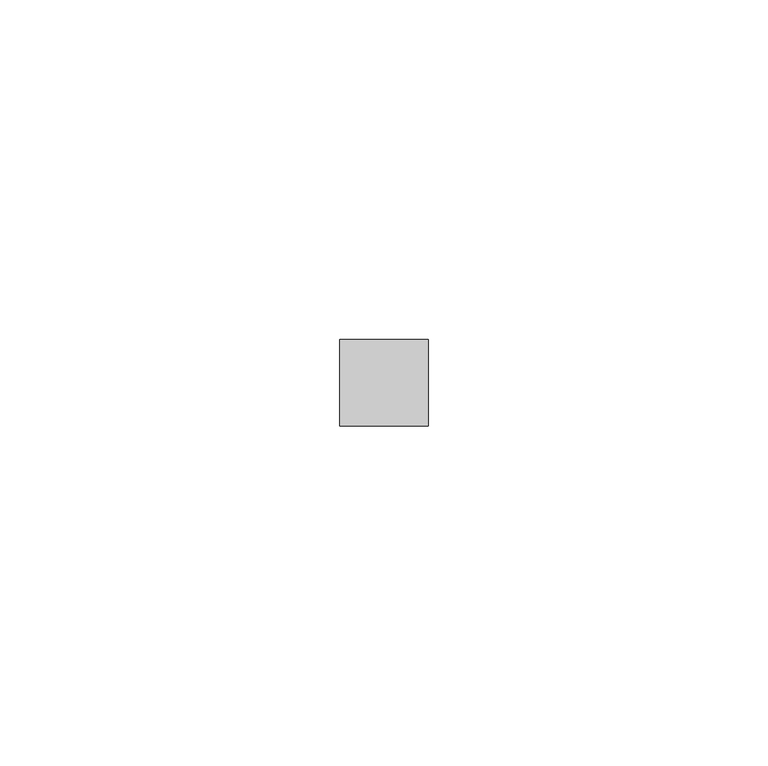
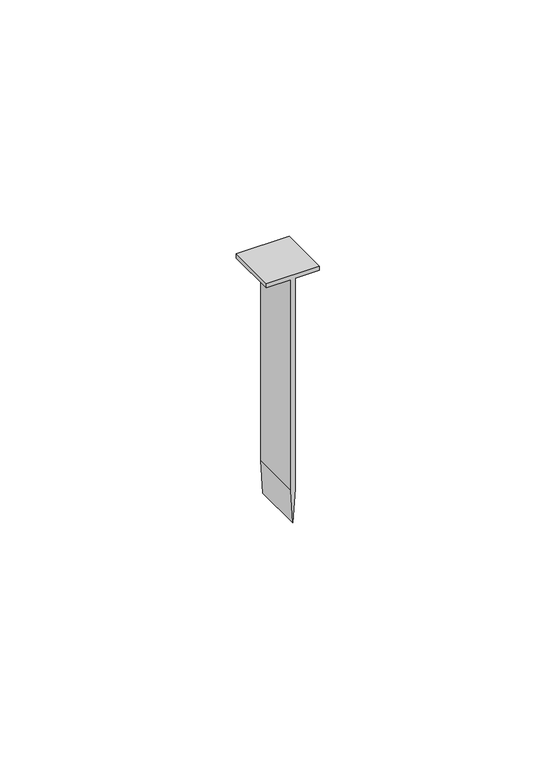
"""IFC4 building model written with IfcOpenShell, lengths in millimetres: proxy geometry, STAINLESS STEEL NAILS009 4160 : STAINLESS STEEL NAILS009 4160."""

from ifc_helpers import new_model, si_unit, frame, origin, place, context, project, spatial, polyline, outline, extrude, source, transform, mapped, element, save


def generic_models_9cc815fe(model_context):
    return source(origin(), model_context, "Body", "SweptSolid", [
        extrude(outline(polyline([(40259.5998489, -2718.4937305), (40259.5998489, -2712.5361379), (40205.2737053, -2712.5361379), (40196.608116, -2711.9945386), (40205.2737053, -2711.4529393), (40259.5998489, -2711.4529393), (40259.5998489, -2705.4953467), (40260.6830476, -2705.4953467), (40260.6830476, -2718.4937305), (40259.5998489, -2718.4937305)])), frame((0.0, -1065.5906573, 0.0), z_axis=(0.0, 1.0, 0.0), x_axis=(0.0, 0.0, 1.0)), (0.0, 0.0, 1.0), 12.7),
    ])


if __name__ == "__main__":
    model = new_model("IFC4")
    model_context = context("Model", 3, world=origin())
    ifc_project = project(units=[si_unit("LENGTHUNIT", "METRE", prefix="MILLI")], contexts=[model_context])
    site = spatial("IfcSite", under=ifc_project)
    building = spatial("IfcBuilding", under=site)
    placement = place(None, origin())
    generic_models_shape = generic_models_9cc815fe(model_context)
    element("IfcBuildingElementProxy", 1, Name="STAINLESS STEEL NAILS009 4160 : STAINLESS STEEL NAILS009 4160", ObjectType="STAINLESS STEEL NAILS009 4160 : STAINLESS STEEL NAILS009 4160", at=placement, inside=building, context=model_context, shape_type="MappedRepresentation", body=[
        mapped(generic_models_shape, transform((0.0, 0.0, 0.0), x_axis=(1.0, 0.0, 0.0), y_axis=(0.0, 1.0, 0.0), z_axis=(0.0, 0.0, 1.0))),
    ])
    save(model, "model.ifc")

# Revit data of these elements
# Type "STAINLESS STEEL NAILS009 4160 : STAINLESS STEEL NAILS009 4160"
#   NameOverride = "STAINLESS STEEL NAILS009"
# Element 1 (IfcBuildingElementProxy, "STAINLESS STEEL NAILS009 4160 : STAINLESS STEEL NAILS009 4160")
#   Materials on its faces: "1 3/4\" STAINLESS STEEL RINGSHANK 5D COMMON NAILS @ 4\" (101.6MM) O.C. FIRESTONE PROVIDED MAX., 1/2\" STAGGERED"
# Materials
#   "1 3/4\" STAINLESS STEEL RINGSHANK 5D COMMON NAILS @ 4\" (101.6MM) O.C. FIRESTONE PROVIDED MAX., 1/2\" STAGGERED": class "Unassigned", colour RGB 255 255 255, transparency 0
